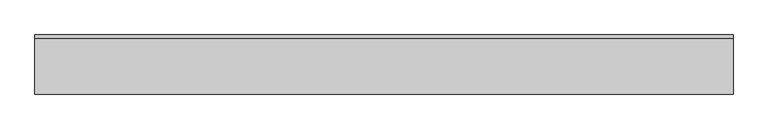
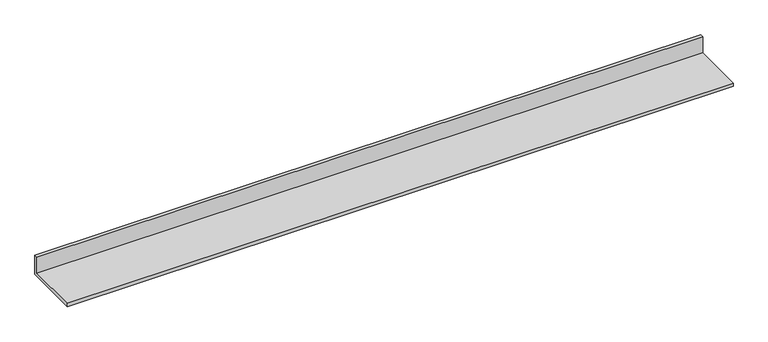
"""IFC4 building model written with IfcOpenShell, lengths in millimetres: proxy geometry, 거터3 : 거터2."""

import ifcopenshell
import ifcopenshell.guid

model = None  # the IFC model being written
_history = None  # IfcOwnerHistory: only IFC2X3 demands one
_inside = {}  # id of a spatial element -> (the spatial element, [elements in it])
_under = {}  # id of a project, library or spatial element -> (it, [spatial elements below it])
_declared = {}  # id of a project -> (the project, [libraries it declares])
_typed = {}  # id of a type object -> (the type object, [elements of that type])
_made_of = {}  # id of a material, layer set ... -> (it, [elements and type objects made of it])


def new_model(schema):
    """Start an empty IFC model of exactly this schema.

    Asked for "IFC4X3", IfcOpenShell would pick the latest addendum, in which some entities
    have other attributes; the version numbers below select the first issue.
    IFC2X3 requires an IfcOwnerHistory on every rooted entity: one is made here for all.
    """
    global model, _history
    if schema == "IFC4X3":
        model = ifcopenshell.file(schema_version=(4, 3, 0, 0))
    else:
        model = ifcopenshell.file(schema=schema)
    _inside.clear()
    _under.clear()
    _declared.clear()
    _typed.clear()
    _made_of.clear()
    _history = None
    if model.schema == "IFC2X3":
        org = make("IfcOrganization", Name="unknown")
        user = make(
            "IfcPersonAndOrganization",
            ThePerson=make("IfcPerson", FamilyName="unknown"),
            TheOrganization=org,
        )
        app = make(
            "IfcApplication",
            ApplicationDeveloper=org,
            Version="unknown",
            ApplicationFullName="unknown",
            ApplicationIdentifier="unknown",
        )
        _history = make(
            "IfcOwnerHistory",
            OwningUser=user,
            OwningApplication=app,
            ChangeAction="ADDED",
            CreationDate=0,
        )
    return model


def make(cls, **values):
    """One entity of the class cls with the attributes given. An attribute that is None is left unset."""
    return model.create_entity(
        cls, **{name: value for name, value in values.items() if value is not None}
    )


def rooted(cls, **values):
    """An entity with a GlobalId (a new one), such as an element, a storey or a relation."""
    return make(cls, GlobalId=ifcopenshell.guid.new(), OwnerHistory=_history, **values)


def si_unit(unit_type, name, prefix=None):
    """IfcSIUnit, for example si_unit("LENGTHUNIT", "METRE", prefix="MILLI")."""
    return make("IfcSIUnit", UnitType=unit_type, Prefix=prefix, Name=name)


def assignment(units):
    """IfcUnitAssignment: the units of a project."""
    return None if units is None else make("IfcUnitAssignment", Units=units)


def point(xyz):
    """IfcCartesianPoint."""
    return None if xyz is None else make("IfcCartesianPoint", Coordinates=xyz)


def direction(xyz):
    """IfcDirection."""
    return None if xyz is None else make("IfcDirection", DirectionRatios=xyz)


def frame(location, z_axis=None, x_axis=None):
    """IfcAxis2Placement3D, a coordinate frame: its origin and axes. An axis left out is left unset."""
    return make(
        "IfcAxis2Placement3D",
        Location=point(location),
        Axis=direction(z_axis),
        RefDirection=direction(x_axis),
    )


def origin():
    """The frame at (0, 0, 0) with its axes left unset."""
    return frame((0.0, 0.0, 0.0))


def place(relative_to, where):
    """IfcLocalPlacement: puts the frame where relative to a parent placement (None: the world)."""
    return make(
        "IfcLocalPlacement", PlacementRelTo=relative_to, RelativePlacement=where
    )


def context(
    kind, dimensions, precision=None, world=None, true_north=None, identifier=None
):
    """IfcGeometricRepresentationContext, for example the 3D "Model" context."""
    return make(
        "IfcGeometricRepresentationContext",
        ContextIdentifier=identifier,
        ContextType=kind,
        CoordinateSpaceDimension=dimensions,
        Precision=precision,
        WorldCoordinateSystem=world,
        TrueNorth=true_north,
    )


def project(units=None, contexts=None):
    """IfcProject with its units and contexts."""
    return rooted(
        "IfcProject",
        Name="project",
        RepresentationContexts=contexts,
        UnitsInContext=assignment(units),
    )


def spatial(cls, under=None, at=None, **own):
    """A site, building, storey or space (cls), placed at a placement, below another one or the project."""
    s = rooted(cls, ObjectPlacement=at, **own)
    if under is not None:
        _under.setdefault(under.id(), (under, []))[1].append(s)
    return s


def polyline(points):
    """IfcPolyline through the points."""
    return make("IfcPolyline", Points=[point(p) for p in points])


def outline(outer, holes=None, kind="AREA"):
    """IfcArbitraryClosedProfileDef: a profile drawn as a closed curve; with holes, ...WithVoids."""
    if holes is None:
        return make("IfcArbitraryClosedProfileDef", ProfileType=kind, OuterCurve=outer)
    return make(
        "IfcArbitraryProfileDefWithVoids",
        ProfileType=kind,
        OuterCurve=outer,
        InnerCurves=holes,
    )


def extrude(swept, where, along, depth):
    """IfcExtrudedAreaSolid: the profile swept, set in the frame where, extruded along a direction by depth."""
    return make(
        "IfcExtrudedAreaSolid",
        SweptArea=swept,
        Position=where,
        ExtrudedDirection=direction(along),
        Depth=depth,
    )


def shape(context_of_items, identifier, shape_type, items):
    """IfcShapeRepresentation: the items that make up one representation, for example the "Body"."""
    return make(
        "IfcShapeRepresentation",
        ContextOfItems=context_of_items,
        RepresentationIdentifier=identifier,
        RepresentationType=shape_type,
        Items=items,
    )


def source(mapping_origin, context_of_items, identifier, shape_type, items):
    """IfcRepresentationMap: a shape defined once, which mapped items show again and again."""
    return make(
        "IfcRepresentationMap",
        MappingOrigin=mapping_origin,
        MappedRepresentation=shape(context_of_items, identifier, shape_type, items),
    )


def transform(
    local_origin,
    x_axis=None,
    y_axis=None,
    z_axis=None,
    scale=None,
    scale2=None,
    scale3=None,
    uniform=True,
):
    """IfcCartesianTransformationOperator3D, or its non-uniform kind. x_axis, y_axis, z_axis: its Axis1, 2, 3."""
    if uniform:
        return make(
            "IfcCartesianTransformationOperator3D",
            Axis1=direction(x_axis),
            Axis2=direction(y_axis),
            LocalOrigin=point(local_origin),
            Scale=scale,
            Axis3=direction(z_axis),
        )
    return make(
        "IfcCartesianTransformationOperator3DnonUniform",
        Axis1=direction(x_axis),
        Axis2=direction(y_axis),
        LocalOrigin=point(local_origin),
        Scale=scale,
        Axis3=direction(z_axis),
        Scale2=scale2,
        Scale3=scale3,
    )


def mapped(mapping_source, mapping_target):
    """IfcMappedItem: shows the shape of a source again, moved by a transform."""
    return make(
        "IfcMappedItem", MappingSource=mapping_source, MappingTarget=mapping_target
    )


def made_of(thing, what):
    """Note that an element or type object is made of a material, layer set ...; save() writes the relation."""
    if what is not None:
        _made_of.setdefault(what.id(), (what, []))[1].append(thing)
    return thing


def element(
    cls,
    number,
    at=None,
    inside=None,
    cuts=None,
    type_object=None,
    material=None,
    context=None,
    identifier="Body",
    shape_type=None,
    held_by="IfcProductDefinitionShape",
    body=None,
    shapes=None,
    **own,
):
    """One element of the class cls, such as IfcWall. Its Tag is "e" and its number.

    at: its placement. inside: the storey or other place that contains it. cuts: it is an
    opening in that element (IfcRelVoidsElement). A single representation is given by context,
    identifier, shape_type and body (its items); several are given by shapes. held_by: the class
    of the entity that holds the representations. save() writes the other relations.
    """
    e = rooted(cls, Tag="e%d" % number, ObjectPlacement=at, **own)
    if body is not None:
        shapes = [shape(context, identifier, shape_type, body)]
    if shapes is not None:
        e.Representation = make(held_by, Representations=shapes)
    if inside is not None:
        _inside.setdefault(inside.id(), (inside, []))[1].append(e)
    if cuts is not None:
        rooted(
            "IfcRelVoidsElement", RelatingBuildingElement=cuts, RelatedOpeningElement=e
        )
    if type_object is not None:
        _typed.setdefault(type_object.id(), (type_object, []))[1].append(e)
    return made_of(e, material)


def aggregate(whole, parts):
    """IfcRelAggregates: a whole, such as a stair, and the parts it consists of."""
    return rooted("IfcRelAggregates", RelatingObject=whole, RelatedObjects=parts)


def save(model, path):
    """Write the relations noted so far, then the file.

    IfcRelAggregates (storeys below a building ...), IfcRelContainedInSpatialStructure (elements
    in a storey), IfcRelDefinesByType, IfcRelAssociatesMaterial and IfcRelDeclares: one each for
    every whole, place, type object, material and project.
    """
    for whole, parts in _under.values():
        aggregate(whole, parts)
    for where, things in _inside.values():
        rooted(
            "IfcRelContainedInSpatialStructure",
            RelatedElements=things,
            RelatingStructure=where,
        )
    for kind, things in _typed.values():
        rooted("IfcRelDefinesByType", RelatedObjects=things, RelatingType=kind)
    for what, things in _made_of.values():
        rooted("IfcRelAssociatesMaterial", RelatedObjects=things, RelatingMaterial=what)
    for by, libraries in _declared.values():
        rooted("IfcRelDeclares", RelatingContext=by, RelatedDefinitions=libraries)
    model.write(path)


def generic_models_a722396c(model_context):
    return source(origin(), model_context, "Body", "SweptSolid", [
        extrude(outline(polyline([(20999.5208589, 6299.9720055), (20159.5208589, 6299.9720055), (20159.5208589, 6349.9720055), (20949.5208589, 6349.9720055), (20949.5208589, 6599.2986846), (20999.5208589, 6599.2986846), (20999.5208589, 6299.9720055)])), frame((40675.0, 0.0, 0.0), z_axis=(1.0, 0.0, 0.0), x_axis=(0.0, 1.0, 0.0)), (0.0, 0.0, 1.0), 9925.0),
    ])


if __name__ == "__main__":
    model = new_model("IFC4")
    model_context = context("Model", 3, world=origin())
    ifc_project = project(units=[si_unit("LENGTHUNIT", "METRE", prefix="MILLI")], contexts=[model_context])
    site = spatial("IfcSite", under=ifc_project)
    building = spatial("IfcBuilding", under=site)
    placement = place(None, origin())
    generic_models_shape = generic_models_a722396c(model_context)
    element("IfcBuildingElementProxy", 1, Name="거터3 : 거터2", ObjectType="거터3 : 거터2", at=placement, inside=building, context=model_context, shape_type="MappedRepresentation", body=[
        mapped(generic_models_shape, transform((0.0, 0.0, 0.0), x_axis=(1.0, 0.0, 0.0), y_axis=(0.0, 1.0, 0.0), z_axis=(0.0, 0.0, 1.0))),
    ])
    save(model, "model.ifc")
